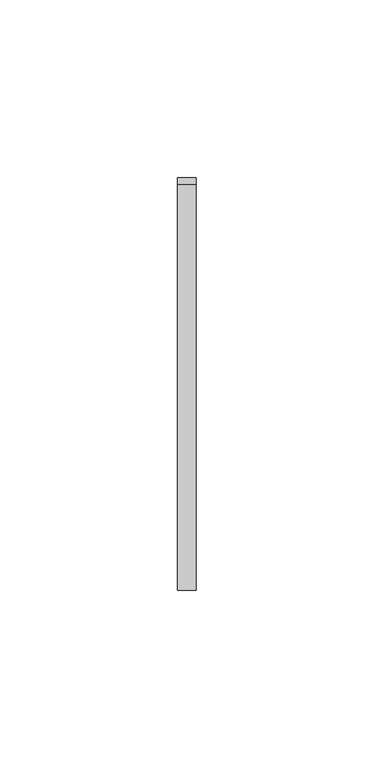
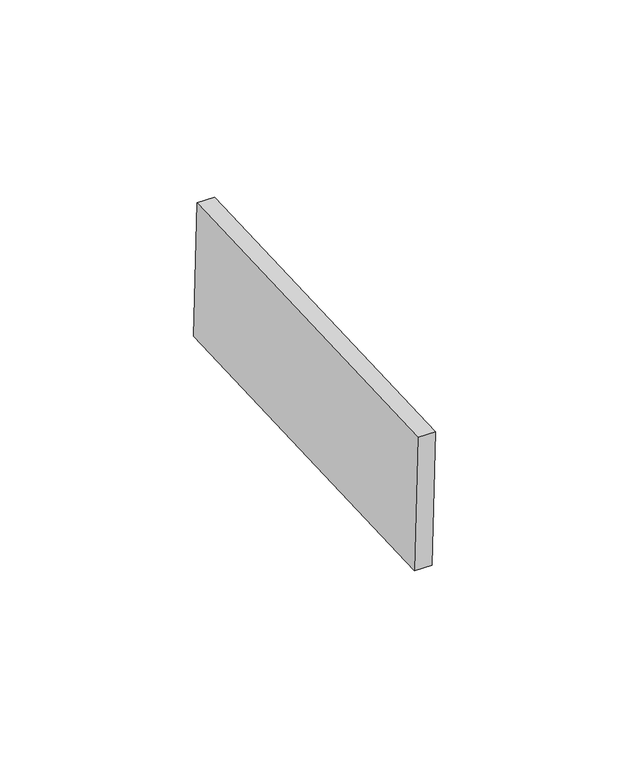
"""IFC4 building model written with IfcOpenShell, lengths in millimetres: proxy geometry, Inner panel:Inner panel:1:Inner panel:1 : Inner panel:Inner panel:300324:2:Inner panel:1:Inner panel:1 : Inner panel:Inner panel:300324:2 : Inner panel:Inner panel:1:Inner panel:1 : Inner panel:Inner panel:300324:300043:68 : Inner panel:Inner panel:1:Inner panel:1 : Inner panel:Inner panel:300324:2:Inner panel:1:Inner panel:1 : Inner panel:Inner panel:300324:2 : Inner panel:Inner panel:1:Inner panel:1 : Inner panel:Inner panel:300324:300043:308120."""

import ifcopenshell
import ifcopenshell.guid

model = None  # the IFC model being written
_history = None  # IfcOwnerHistory: only IFC2X3 demands one
_inside = {}  # id of a spatial element -> (the spatial element, [elements in it])
_under = {}  # id of a project, library or spatial element -> (it, [spatial elements below it])
_declared = {}  # id of a project -> (the project, [libraries it declares])
_typed = {}  # id of a type object -> (the type object, [elements of that type])
_made_of = {}  # id of a material, layer set ... -> (it, [elements and type objects made of it])


def new_model(schema):
    """Start an empty IFC model of exactly this schema.

    Asked for "IFC4X3", IfcOpenShell would pick the latest addendum, in which some entities
    have other attributes; the version numbers below select the first issue.
    IFC2X3 requires an IfcOwnerHistory on every rooted entity: one is made here for all.
    """
    global model, _history
    if schema == "IFC4X3":
        model = ifcopenshell.file(schema_version=(4, 3, 0, 0))
    else:
        model = ifcopenshell.file(schema=schema)
    _inside.clear()
    _under.clear()
    _declared.clear()
    _typed.clear()
    _made_of.clear()
    _history = None
    if model.schema == "IFC2X3":
        org = make("IfcOrganization", Name="unknown")
        user = make(
            "IfcPersonAndOrganization",
            ThePerson=make("IfcPerson", FamilyName="unknown"),
            TheOrganization=org,
        )
        app = make(
            "IfcApplication",
            ApplicationDeveloper=org,
            Version="unknown",
            ApplicationFullName="unknown",
            ApplicationIdentifier="unknown",
        )
        _history = make(
            "IfcOwnerHistory",
            OwningUser=user,
            OwningApplication=app,
            ChangeAction="ADDED",
            CreationDate=0,
        )
    return model


def make(cls, **values):
    """One entity of the class cls with the attributes given. An attribute that is None is left unset."""
    return model.create_entity(
        cls, **{name: value for name, value in values.items() if value is not None}
    )


def rooted(cls, **values):
    """An entity with a GlobalId (a new one), such as an element, a storey or a relation."""
    return make(cls, GlobalId=ifcopenshell.guid.new(), OwnerHistory=_history, **values)


def si_unit(unit_type, name, prefix=None):
    """IfcSIUnit, for example si_unit("LENGTHUNIT", "METRE", prefix="MILLI")."""
    return make("IfcSIUnit", UnitType=unit_type, Prefix=prefix, Name=name)


def assignment(units):
    """IfcUnitAssignment: the units of a project."""
    return None if units is None else make("IfcUnitAssignment", Units=units)


def point(xyz):
    """IfcCartesianPoint."""
    return None if xyz is None else make("IfcCartesianPoint", Coordinates=xyz)


def direction(xyz):
    """IfcDirection."""
    return None if xyz is None else make("IfcDirection", DirectionRatios=xyz)


def frame(location, z_axis=None, x_axis=None):
    """IfcAxis2Placement3D, a coordinate frame: its origin and axes. An axis left out is left unset."""
    return make(
        "IfcAxis2Placement3D",
        Location=point(location),
        Axis=direction(z_axis),
        RefDirection=direction(x_axis),
    )


def origin():
    """The frame at (0, 0, 0) with its axes left unset."""
    return frame((0.0, 0.0, 0.0))


def place(relative_to, where):
    """IfcLocalPlacement: puts the frame where relative to a parent placement (None: the world)."""
    return make(
        "IfcLocalPlacement", PlacementRelTo=relative_to, RelativePlacement=where
    )


def context(
    kind, dimensions, precision=None, world=None, true_north=None, identifier=None
):
    """IfcGeometricRepresentationContext, for example the 3D "Model" context."""
    return make(
        "IfcGeometricRepresentationContext",
        ContextIdentifier=identifier,
        ContextType=kind,
        CoordinateSpaceDimension=dimensions,
        Precision=precision,
        WorldCoordinateSystem=world,
        TrueNorth=true_north,
    )


def project(units=None, contexts=None):
    """IfcProject with its units and contexts."""
    return rooted(
        "IfcProject",
        Name="project",
        RepresentationContexts=contexts,
        UnitsInContext=assignment(units),
    )


def spatial(cls, under=None, at=None, **own):
    """A site, building, storey or space (cls), placed at a placement, below another one or the project."""
    s = rooted(cls, ObjectPlacement=at, **own)
    if under is not None:
        _under.setdefault(under.id(), (under, []))[1].append(s)
    return s


def polyline(points):
    """IfcPolyline through the points."""
    return make("IfcPolyline", Points=[point(p) for p in points])


def outline(outer, holes=None, kind="AREA"):
    """IfcArbitraryClosedProfileDef: a profile drawn as a closed curve; with holes, ...WithVoids."""
    if holes is None:
        return make("IfcArbitraryClosedProfileDef", ProfileType=kind, OuterCurve=outer)
    return make(
        "IfcArbitraryProfileDefWithVoids",
        ProfileType=kind,
        OuterCurve=outer,
        InnerCurves=holes,
    )


def extrude(swept, where, along, depth):
    """IfcExtrudedAreaSolid: the profile swept, set in the frame where, extruded along a direction by depth."""
    return make(
        "IfcExtrudedAreaSolid",
        SweptArea=swept,
        Position=where,
        ExtrudedDirection=direction(along),
        Depth=depth,
    )


def shape(context_of_items, identifier, shape_type, items):
    """IfcShapeRepresentation: the items that make up one representation, for example the "Body"."""
    return make(
        "IfcShapeRepresentation",
        ContextOfItems=context_of_items,
        RepresentationIdentifier=identifier,
        RepresentationType=shape_type,
        Items=items,
    )


def source(mapping_origin, context_of_items, identifier, shape_type, items):
    """IfcRepresentationMap: a shape defined once, which mapped items show again and again."""
    return make(
        "IfcRepresentationMap",
        MappingOrigin=mapping_origin,
        MappedRepresentation=shape(context_of_items, identifier, shape_type, items),
    )


def transform(
    local_origin,
    x_axis=None,
    y_axis=None,
    z_axis=None,
    scale=None,
    scale2=None,
    scale3=None,
    uniform=True,
):
    """IfcCartesianTransformationOperator3D, or its non-uniform kind. x_axis, y_axis, z_axis: its Axis1, 2, 3."""
    if uniform:
        return make(
            "IfcCartesianTransformationOperator3D",
            Axis1=direction(x_axis),
            Axis2=direction(y_axis),
            LocalOrigin=point(local_origin),
            Scale=scale,
            Axis3=direction(z_axis),
        )
    return make(
        "IfcCartesianTransformationOperator3DnonUniform",
        Axis1=direction(x_axis),
        Axis2=direction(y_axis),
        LocalOrigin=point(local_origin),
        Scale=scale,
        Axis3=direction(z_axis),
        Scale2=scale2,
        Scale3=scale3,
    )


def mapped(mapping_source, mapping_target):
    """IfcMappedItem: shows the shape of a source again, moved by a transform."""
    return make(
        "IfcMappedItem", MappingSource=mapping_source, MappingTarget=mapping_target
    )


def made_of(thing, what):
    """Note that an element or type object is made of a material, layer set ...; save() writes the relation."""
    if what is not None:
        _made_of.setdefault(what.id(), (what, []))[1].append(thing)
    return thing


def element(
    cls,
    number,
    at=None,
    inside=None,
    cuts=None,
    type_object=None,
    material=None,
    context=None,
    identifier="Body",
    shape_type=None,
    held_by="IfcProductDefinitionShape",
    body=None,
    shapes=None,
    **own,
):
    """One element of the class cls, such as IfcWall. Its Tag is "e" and its number.

    at: its placement. inside: the storey or other place that contains it. cuts: it is an
    opening in that element (IfcRelVoidsElement). A single representation is given by context,
    identifier, shape_type and body (its items); several are given by shapes. held_by: the class
    of the entity that holds the representations. save() writes the other relations.
    """
    e = rooted(cls, Tag="e%d" % number, ObjectPlacement=at, **own)
    if body is not None:
        shapes = [shape(context, identifier, shape_type, body)]
    if shapes is not None:
        e.Representation = make(held_by, Representations=shapes)
    if inside is not None:
        _inside.setdefault(inside.id(), (inside, []))[1].append(e)
    if cuts is not None:
        rooted(
            "IfcRelVoidsElement", RelatingBuildingElement=cuts, RelatedOpeningElement=e
        )
    if type_object is not None:
        _typed.setdefault(type_object.id(), (type_object, []))[1].append(e)
    return made_of(e, material)


def aggregate(whole, parts):
    """IfcRelAggregates: a whole, such as a stair, and the parts it consists of."""
    return rooted("IfcRelAggregates", RelatingObject=whole, RelatedObjects=parts)


def save(model, path):
    """Write the relations noted so far, then the file.

    IfcRelAggregates (storeys below a building ...), IfcRelContainedInSpatialStructure (elements
    in a storey), IfcRelDefinesByType, IfcRelAssociatesMaterial and IfcRelDeclares: one each for
    every whole, place, type object, material and project.
    """
    for whole, parts in _under.values():
        aggregate(whole, parts)
    for where, things in _inside.values():
        rooted(
            "IfcRelContainedInSpatialStructure",
            RelatedElements=things,
            RelatingStructure=where,
        )
    for kind, things in _typed.values():
        rooted("IfcRelDefinesByType", RelatedObjects=things, RelatingType=kind)
    for what, things in _made_of.values():
        rooted("IfcRelAssociatesMaterial", RelatedObjects=things, RelatingMaterial=what)
    for by, libraries in _declared.values():
        rooted("IfcRelDeclares", RelatingContext=by, RelatedDefinitions=libraries)
    model.write(path)


def generic_models_c1ce71e3(model_context):
    return source(origin(), model_context, "Body", "SweptSolid", [
        extrude(outline(polyline([(0.0, -114.3), (0.0, 0.0), (5.2138089, 0.0), (5.2138089, -114.3), (0.0, -114.3)])), frame((593936.595117, -578297.797364, 3981.6641254), z_axis=(0.0, -0.04163054471216399, 0.9991330730923527), x_axis=(-1.0, 0.0, 0.0)), (0.0, 0.0, 1.0), 43.2233908),
    ])


if __name__ == "__main__":
    model = new_model("IFC4")
    model_context = context("Model", 3, world=origin())
    ifc_project = project(units=[si_unit("LENGTHUNIT", "METRE", prefix="MILLI")], contexts=[model_context])
    site = spatial("IfcSite", under=ifc_project)
    building = spatial("IfcBuilding", under=site)
    placement = place(None, origin())
    generic_models_shape = generic_models_c1ce71e3(model_context)
    element("IfcBuildingElementProxy", 1, Name="Inner panel:Inner panel:1:Inner panel:1 : Inner panel:Inner panel:300324:2:Inner panel:1:Inner panel:1 : Inner panel:Inner panel:300324:2 : Inner panel:Inner panel:1:Inner panel:1 : Inner panel:Inner panel:300324:300043:68 : Inner panel:Inner panel:1:Inner panel:1 : Inner panel:Inner panel:300324:2:Inner panel:1:Inner panel:1 : Inner panel:Inner panel:300324:2 : Inner panel:Inner panel:1:Inner panel:1 : Inner panel:Inner panel:300324:300043:308120", ObjectType="Inner panel:Inner panel:1:Inner panel:1 : Inner panel:Inner panel:300324:2:Inner panel:1:Inner panel:1 : Inner panel:Inner panel:300324:2 : Inner panel:Inner panel:1:Inner panel:1 : Inner panel:Inner panel:300324:300043:68 : Inner panel:Inner panel:1:Inner panel:1 : Inner panel:Inner panel:300324:2:Inner panel:1:Inner panel:1 : Inner panel:Inner panel:300324:2 : Inner panel:Inner panel:1:Inner panel:1 : Inner panel:Inner panel:300324:300043:308120", at=placement, inside=building, context=model_context, shape_type="MappedRepresentation", body=[
        mapped(generic_models_shape, transform((0.0, 0.0, 0.0), x_axis=(1.0, 0.0, 0.0), y_axis=(0.0, 1.0, 0.0), z_axis=(0.0, 0.0, 1.0))),
    ])
    save(model, "model.ifc")

# Revit data of these elements
# Type "Inner panel:Inner panel:1:Inner panel:1 : Inner panel:Inner panel:300324:2:Inner panel:1:Inner panel:1 : Inner panel:Inner panel:300324:2 : Inner panel:Inner panel:1:Inner panel:1 : Inner panel:Inner panel:300324:300043:68 : Inner panel:Inner panel:1:Inner panel:1 : Inner panel:Inner panel:300324:2:Inner panel:1:Inner panel:1 : Inner panel:Inner panel:300324:2 : Inner panel:Inner panel:1:Inner panel:1 : Inner panel:Inner panel:300324:300043:308120"
#   NameOverride = "Inner panel:Inner panel:1:Inner panel:1 : Inner panel:Inner panel:300324:2:Inner panel:1:Inner panel:1 : Inner panel:Inner panel:300324:2 : Inner panel:Inner panel:1:Inner panel:1 : Inner panel:Inner panel:300324:300043:308120"
#   ObjectTypeOverride = "Inner panel:1:Inner panel:1 : Inner panel:Inner panel:300324:2 : Inner panel:Inner panel:1:Inner panel:1 : Inner panel:Inner panel:300324:300043"
#   Reference = "Inner panel"
#   Tag = "308120"
# Element 1 (IfcBuildingElementProxy, "Inner panel:Inner panel:1:Inner panel:1 : Inner panel:Inner panel:300324:2:Inner panel:1:Inner panel:1 : Inner panel:Inner panel:300324:2 : Inner panel:Inner panel:1:Inner panel:1 : Inner panel:Inner panel:300324:300043:68 : Inner panel:Inner panel:1:Inner panel:1 : Inner panel:Inner panel:300324:2:Inner panel:1:Inner panel:1 : Inner panel:Inner panel:300324:2 : Inner panel:Inner panel:1:Inner panel:1 : Inner panel:Inner panel:300324:300043:308120")
#   Materials on its faces: "SLIDING CLIP"
# Materials
#   "SLIDING CLIP": class "Generic", colour RGB 120 120 120, transparency 0, Cost = 0
